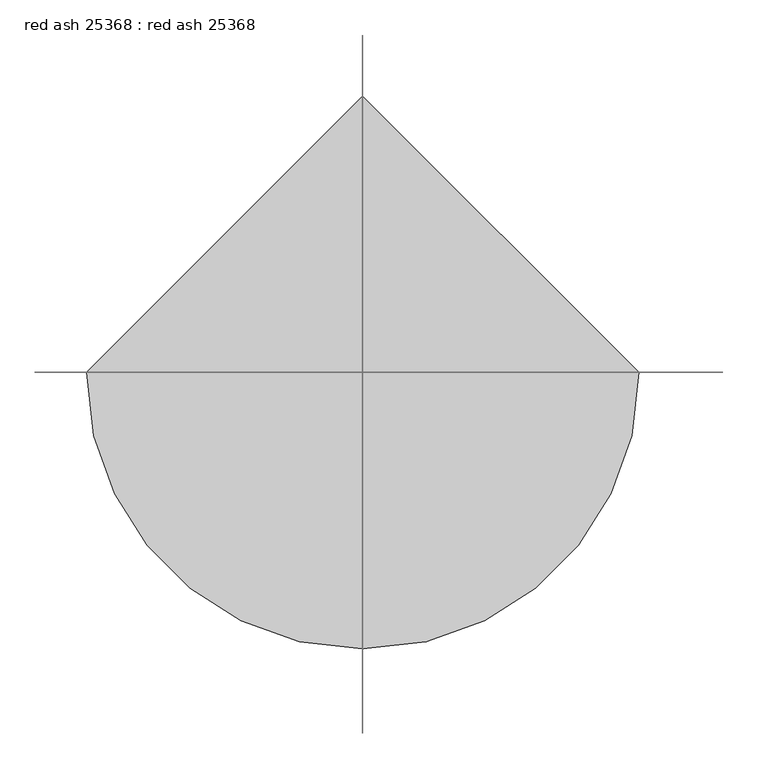
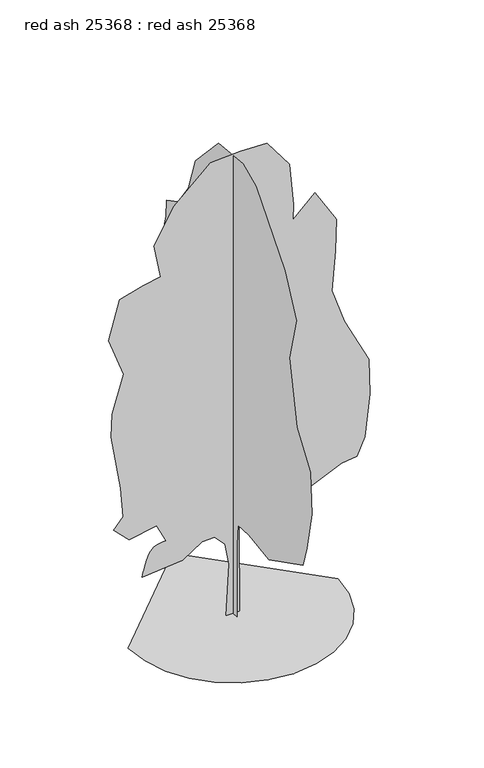
"""IFC4 building model written with IfcOpenShell, lengths in millimetres: proxy geometry, red ash 25368 : red ash 25368."""

from ifc_helpers import new_model, si_unit, origin, place, context, project, spatial, triangles, source, transform, mapped, element, save


def red_ash_25368_red_ash_25368_14781bec(model_context):
    return source(origin(), model_context, "Body", "Tessellation", [
        triangles([(-1644.9525009, 0.0, 6.19e-05), (-1601.4651844, -376.9143482, 6.19e-05), (-1477.6144592, -723.0498339, 6.19e-05), (-1283.3164352, -1028.4894024, 6.19e-05), (-1028.4894751, -1283.3165806, 6.19e-05), (-723.0496885, -1477.6140232, 6.19e-05), (-376.9141665, -1601.4651844, 6.19e-05), (7.19e-05, -1644.9525009, 6.19e-05), (376.9143846, -1601.4651844, 6.19e-05), (723.0499065, -1477.6143139, 6.19e-05), (1028.4894751, -1283.3164352, 6.19e-05), (1283.3168713, -1028.4894751, 6.19e-05), (1477.6141685, -723.0496159, 6.19e-05), (1601.4651844, -376.9140939, 6.19e-05), (1644.9525009, 0.0001438, 6.19e-05), (-0.0002157, 1644.9525009, 6.19e-05), (-1.07e-05, -102.8462569, 0.0), (2.5e-05, -101.2467179, 1194.554048), (3.23e-05, -129.8819613, 1537.8029366), (7e-07, -438.8253948, 1558.1655018), (-5.78e-05, -976.3912743, 1478.3068588), (-0.0001405, -1903.692667, 1948.6771305), (-0.0001413, -2011.2060173, 2298.095192), (-0.0001361, -2145.5975235, 2943.1744217), (-0.0001119, -2105.2803623, 3615.1319527), (-5.81e-05, -1740.3819958, 4141.0172951), (-5.5e-06, -1527.3986298, 5160.6350006), (-3.5e-06, -1715.5451397, 5886.3488434), (4.79e-05, -1406.4449661, 6531.4286545), (0.0001569, -626.9743755, 7458.7301926), (0.0001985, -273.2007115, 7618.1942963), (0.0002662, 394.4016166, 7552.8046829), (0.0003121, 1026.0418774, 6880.8468613), (0.0003149, 1214.190204, 6316.4022446), (0.0003323, 1496.411277, 5913.2274353), (0.0003598, 1805.5131947, 5751.9582092), (0.0003531, 1818.9521999, 5483.1746155), (0.0003523, 1899.587249, 5174.0742966), (0.0003275, 1765.1957428, 4811.2170845), (0.0003297, 1886.1480984, 4461.7991684), (0.0003279, 2007.1004539, 3977.9897461), (0.0003211, 1980.222298, 3843.5979492), (0.0002877, 1751.7567375, 3521.0580437), (0.0002729, 1737.3115437, 3077.5662186), (0.0002632, 1724.8782909, 2795.3439102), (0.0002542, 1738.3174416, 2445.9262848), (0.0002412, 1751.7568829, 1962.1167171), (0.0002172, 1563.6084835, 1814.2857697), (0.0001807, 1214.1907127, 1814.2857697), (0.0001827, 1375.4605202, 1317.0371967), (0.0001715, 1348.4951603, 1034.8845062), (0.0001516, 1103.0310734, 1227.8363914), (9.86e-05, 629.4626684, 1106.7075932), (9.8e-05, 551.7118183, 1357.0609165), (6.29e-05, 215.9127657, 1354.0025276), (5.03e-05, 130.8012366, 1228.3346169), (3.27e-05, 79.5493323, 818.2831198), (1.17e-05, 112.1660096, 1.28e-05), (-110.870867, 4.8e-06, 4.46e-05), (-66.7114758, -9.64e-05, 833.5016676), (-129.3072962, -0.000136, 1187.9435503), (-290.7878647, -0.00015, 1365.31768), (-483.6364677, -0.0001408, 1358.6964272), (-796.2678211, -0.000103, 1155.7673166), (-1427.9080456, -6.9e-05, 1102.0108595), (-1419.1706429, -7.35e-05, 1136.7646975), (-1409.8454853, -7.82e-05, 1172.6938271), (-1399.3449635, -8.32e-05, 1210.9736853), (-1387.0813225, -8.87e-05, 1252.7803631), (-1372.4668076, -9.49e-05, 1299.2876987), (-1354.9136639, -0.0001019, 1351.6733093), (-1333.8341366, -0.0001099, 1411.1111057), (-1307.2693336, -0.0001176, 1466.2392815), (-1274.3570984, -0.0001239, 1506.556588), (-1236.1555058, -0.0001289, 1534.5316246), (-1193.7220493, -0.0001329, 1552.6338627), (-1148.1152401, -0.0001362, 1563.3300121), (-1100.3923536, -0.000139, 1569.0895443), (-1051.6116829, -0.0001415, 1572.3809132), (-1199.4421944, -0.0001703, 1868.0423721), (-1629.4953049, -0.0001418, 1787.4073231), (-1871.3997253, -0.0001601, 2029.3124702), (-1723.5690685, -0.0001874, 2204.0214283), (-1763.886375, -0.0002433, 2687.8309959), (-1911.7170319, -0.0003442, 3588.2539421), (-1898.4807758, -0.0003892, 3961.1654823), (-1719.9175472, -0.0004688, 4563.3255295), (-1952.0346291, -0.0005347, 5200.9523071), (-1777.3253803, -0.000616, 5819.1535263), (-1414.4687496, -0.0006447, 5926.6667313), (-1138.413216, -0.0006626, 5975.3625961), (-1239.7599369, -0.0007228, 6517.9893585), (-930.6591093, -0.000802, 7068.9952606), (-352.7753057, -0.0008898, 7593.1219894), (117.5946844, -0.0009135, 7620.0), (534.2087442, -0.0009301, 7606.5601227), (883.626733, -0.0008893, 7136.1905777), (947.8720848, -0.00081, 6447.5180786), (938.6469212, -0.0007795, 6194.9695404), (1286.8011063, -0.0008333, 6517.9893585), (1622.7800171, -0.0007823, 5966.9840378), (1609.3410118, -0.0007196, 5446.5094116), (1549.4574577, -0.00064, 4800.6520317), (1743.7323727, -0.0005809, 4233.3331718), (2131.7640656, -0.0005067, 3469.1978371), (2144.1354034, -0.0004386, 2892.8094727), (2066.2719875, -0.0003531, 2204.021283), (1945.319632, -0.0003141, 1921.7989746), (1703.4147755, -0.0003004, 1894.9206734), (1233.0446491, -0.0002542, 1679.8941181), (816.4305439, -0.0002007, 1384.2328045), (257.4765441, -0.0002049, 1624.5688614), (93.0508701, -0.0001766, 1447.6347485), (104.1552431, -4.6e-06, 3.52e-05)], [[15, 16, 1], [14, 15, 1], [14, 1, 2], [13, 14, 2], [13, 2, 3], [13, 3, 4], [12, 13, 4], [11, 12, 4], [11, 4, 5], [11, 5, 6], [11, 6, 7], [11, 7, 8], [11, 8, 9], [11, 9, 10], [50, 51, 52], [57, 58, 17], [57, 17, 18], [56, 57, 18], [56, 18, 19], [55, 56, 19], [49, 50, 52], [52, 53, 54], [49, 52, 54], [35, 36, 37], [46, 47, 48], [46, 48, 49], [21, 22, 23], [20, 21, 23], [20, 23, 24], [20, 24, 25], [20, 25, 26], [19, 20, 26], [19, 26, 27], [45, 46, 49], [31, 32, 33], [30, 31, 33], [29, 30, 33], [29, 33, 34], [28, 29, 34], [27, 28, 34], [19, 27, 34], [19, 34, 35], [19, 35, 37], [19, 37, 38], [19, 38, 39], [19, 39, 40], [19, 40, 41], [19, 41, 42], [19, 42, 43], [19, 43, 44], [19, 44, 45], [19, 45, 49], [19, 49, 54], [55, 19, 54], [64, 65, 66], [64, 66, 67], [64, 67, 68], [99, 100, 101], [64, 68, 69], [64, 69, 70], [64, 70, 71], [114, 59, 60], [113, 114, 60], [113, 60, 61], [113, 61, 62], [64, 71, 72], [64, 72, 73], [64, 73, 74], [64, 74, 75], [64, 75, 76], [64, 76, 77], [64, 77, 78], [64, 78, 79], [63, 64, 79], [81, 82, 83], [80, 81, 83], [99, 101, 102], [107, 108, 109], [110, 111, 112], [88, 89, 90], [87, 88, 90], [87, 90, 91], [80, 83, 84], [95, 96, 97], [95, 97, 98], [94, 95, 98], [93, 94, 98], [92, 93, 98], [91, 92, 98], [91, 98, 99], [87, 91, 99], [87, 99, 102], [87, 102, 103], [87, 103, 104], [86, 87, 104], [85, 86, 104], [84, 85, 104], [80, 84, 104], [80, 104, 105], [80, 105, 106], [80, 106, 107], [80, 107, 109], [80, 109, 110], [80, 110, 112], [79, 80, 112], [63, 79, 112], [62, 63, 112], [113, 62, 112]], closed=False),
    ])


if __name__ == "__main__":
    model = new_model("IFC4")
    model_context = context("Model", 3, world=origin())
    ifc_project = project(units=[si_unit("LENGTHUNIT", "METRE", prefix="MILLI")], contexts=[model_context])
    site = spatial("IfcSite", under=ifc_project)
    building = spatial("IfcBuilding", under=site)
    placement = place(None, origin())
    red_ash_25368_red_ash_25368_shape = red_ash_25368_red_ash_25368_14781bec(model_context)
    element("IfcBuildingElementProxy", 1, Name="red ash 25368 : red ash 25368", ObjectType="red ash 25368 : red ash 25368", at=placement, inside=building, context=model_context, shape_type="MappedRepresentation", body=[
        mapped(red_ash_25368_red_ash_25368_shape, transform((0.0, 0.0, 0.0), x_axis=(1.0, 0.0, 0.0), y_axis=(0.0, 1.0, 0.0), z_axis=(0.0, 0.0, 1.0))),
    ])
    save(model, "model.ifc")

# Revit data of these elements
# Type "red ash 25368 : red ash 25368"
#   built-in parameter 1005195 = "RPC-8-G3GR-497X-PHW5-6"
#   Height = 0
